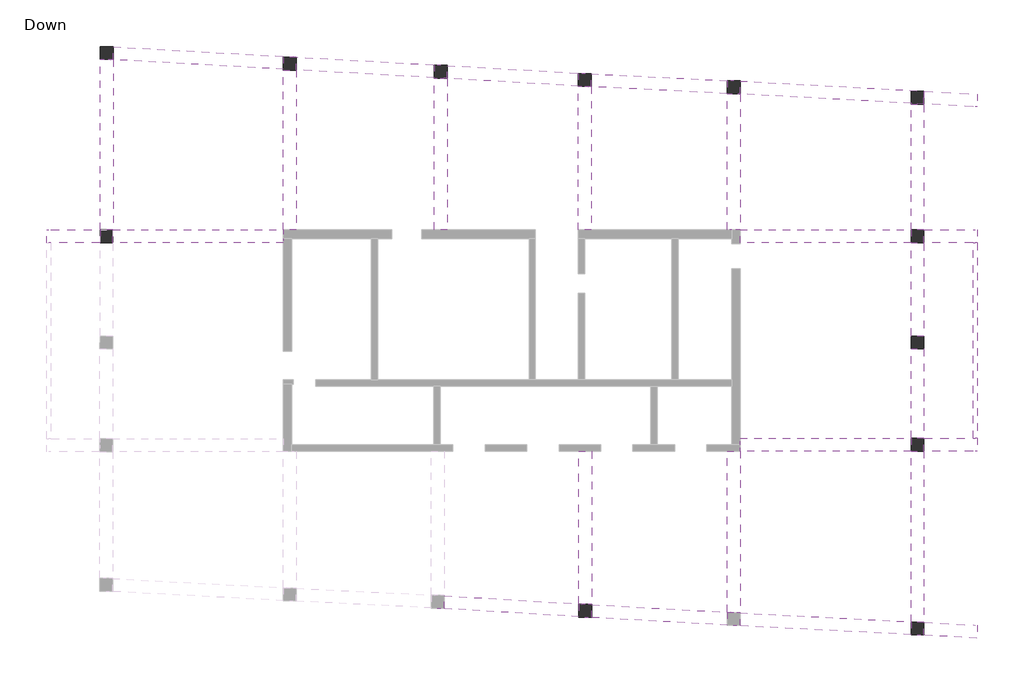
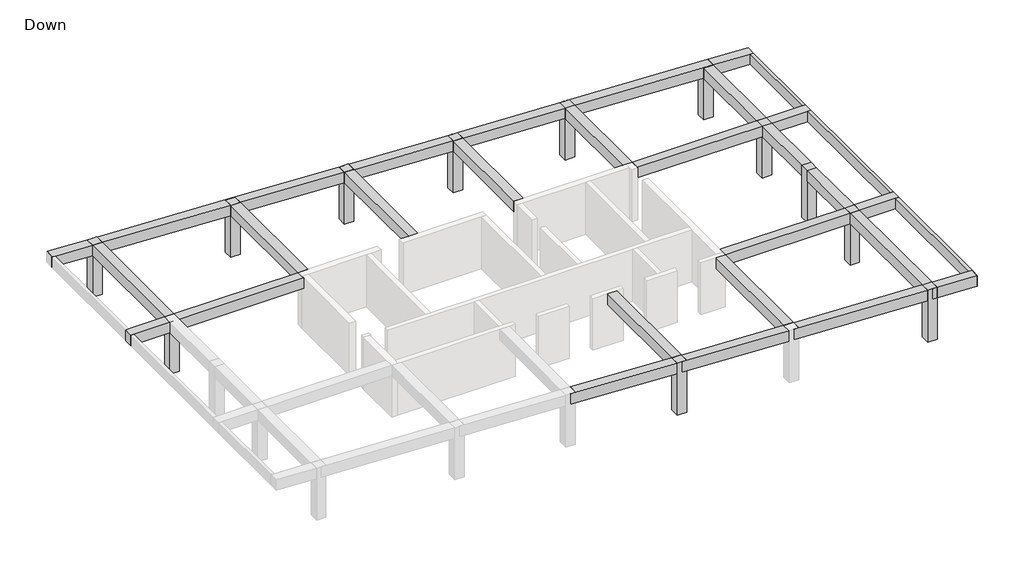
# One storey, part 2 of 2: 28 beams, 12 columns.
"""IFC4 building model written with IfcOpenShell, lengths in millimetres."""

from ifc_helpers import new_model, si_unit, origin, origin_with_axes, place, context, project, spatial, polyline, outline, extrude, faceted_brep, element, save

model = new_model("IFC4")

# Units and contexts
model_context = context("Model", 3, world=origin())
ifc_project = project(units=[si_unit("LENGTHUNIT", "METRE", prefix="MILLI")], contexts=[model_context])

# Site, building, storey
site = spatial("IfcSite", under=ifc_project)
building = spatial("IfcBuilding", under=site)
storey = spatial("IfcBuildingStorey", under=building, Name="Down", Elevation=0.0)

# Beams
placement = place(None, origin())
element("IfcBeam", 1, ObjectType="Concrete Rectengular Beam : 20/70", at=placement, inside=storey, context=model_context, shape_type="Brep", body=[
    faceted_brep([(24768.7448881, 7874.5583517, 3500.0), (24568.7448881, 7885.5038131, 3500.0), (24568.7448881, 2137.8533878, 3500.0), (24768.7448881, 2137.8533878, 3500.0), (24768.7448881, 7874.5583517, 2800.0), (24768.7448881, 2137.8533878, 2800.0), (24568.7448881, 7885.5038131, 2800.0), (24568.7448881, 2137.8533878, 2800.0), (24568.7448881, 7885.5038131, 3250.0), (24568.7448881, 2137.8533878, 3250.0)], [[[0, 1, 2, 3]], [[4, 0, 3, 5]], [[6, 4, 5, 7]], [[1, 8, 6, 7, 9, 2]], [[1, 0, 4, 6, 8]], [[3, 2, 9, 7, 5]]]),
    faceted_brep([(24768.7448881, -16893.2994445, 2800.0), (24768.7448881, -16893.2994445, 3500.0), (24737.8761026, -16891.709202, 3500.0), (24737.8761026, -16891.709202, 2800.0), (24768.7448881, -16292.5037964, 2800.0), (24768.7448881, -16292.5037964, 3500.0), (24568.7448881, -16282.2005564, 3500.0), (24568.7448881, -16282.2005564, 3250.0), (24568.7448881, -16282.2005564, 2800.0), (24568.7448881, -8172.2965545, 3500.0), (24768.7448881, -8172.2965545, 3500.0), (24768.7448881, -8172.2965545, 2800.0), (24568.7448881, -8172.2965545, 2800.0), (24568.7448881, -8172.2965545, 3250.0)], [[[0, 1, 2, 3]], [[4, 5, 6, 7, 8]], [[5, 4, 3, 2]], [[2, 1, 5]], [[0, 3, 4]], [[9, 10, 11, 12, 13]], [[6, 5, 10, 9]], [[1, 0, 4, 11, 10, 5]], [[4, 8, 12, 11]], [[8, 7, 6, 9, 13, 12]]]),
    faceted_brep([(24768.7448881, -7572.2965545, 3500.0), (24568.7448881, -7572.2965545, 3500.0), (24568.7448881, -7572.2965545, 3250.0), (24568.7448881, -7572.2965545, 2800.0), (24768.7448881, -7572.2965545, 2800.0), (24568.7448881, 1537.8533878, 3500.0), (24768.7448881, 1537.8533878, 3500.0), (24768.7448881, 1537.8533878, 2800.0), (24568.7448881, 1537.8533878, 2800.0), (24568.7448881, 1537.8533878, 3250.0)], [[[0, 1, 2, 3, 4]], [[5, 6, 7, 8, 9]], [[1, 0, 6, 5]], [[0, 4, 7, 6]], [[4, 3, 8, 7]], [[3, 2, 1, 5, 9, 8]]]),
])
element("IfcBeam", 2, ObjectType="Concrete Rectengular Beam : 60/70", at=placement, inside=storey, context=model_context, shape_type="Brep", body=[
    faceted_brep([(-15535.8201837, 10679.5964096, 3500.0), (-15536.4529131, 10091.1580694, 3500.0), (-15762.4756779, 10091.4011046, 3500.0), (-15536.4663265, 10078.6836364, 3500.0), (-7599.5626242, 9632.0768029, 3500.0), (-7599.5626242, 10196.3425232, 3500.0), (-6999.5626242, 10196.3425232, 3500.0), (-6999.5626242, 10199.2641414, 3500.0), (-7278.9210368, 10214.9835429, 3500.0), (-15762.4756779, 10091.4011046, 2800.0), (-15536.4663265, 10078.6836364, 2800.0), (-7599.5626242, 9632.0768029, 2800.0), (-7599.5626242, 9632.0768029, 3250.0), (-15536.4529131, 10091.1580694, 2800.0), (-15535.8201837, 10679.5964096, 2800.0), (-7278.9210368, 10214.9835429, 2800.0), (-6999.5626242, 10199.2641414, 2800.0), (-6999.5626242, 10196.3425232, 2800.0), (-7599.5626242, 10196.3425232, 2800.0)], [[[0, 1, 2, 3, 4, 5, 6, 7, 8]], [[2, 9, 10, 11, 12, 4, 3]], [[13, 14, 15, 16, 17, 18, 11, 10, 9]], [[14, 0, 8, 7, 16, 15]], [[1, 0, 14, 13]], [[1, 13, 9, 2]], [[5, 4, 12, 11, 18]], [[5, 18, 17, 6]], [[16, 7, 6, 17]]]),
    faceted_brep([(-16135.8074053, 10691.8028834, 2800.0), (-16135.8074053, 10691.8028834, 3500.0), (-16136.4303725, 10112.4434063, 3500.0), (-16136.4303725, 10112.4434063, 3250.0), (-16136.4303725, 10112.4434063, 2800.0), (-15745.2858019, 10691.3829677, 2800.0), (-15745.2858019, 10691.3829677, 3500.0), (-18643.7818749, 10253.5312104, 3500.0), (-18643.7818749, 10253.5312104, 2800.0), (-18443.7818749, 10242.2772794, 2800.0), (-18443.7818749, 10242.2772794, 3500.0), (-18610.0734048, 10852.5835779, 3500.0), (-18610.0734048, 10852.5835779, 2800.0)], [[[0, 1, 2, 3, 4]], [[1, 0, 5, 6]], [[7, 8, 9, 4, 3, 2, 10]], [[11, 12, 8, 7]], [[2, 1, 6, 11, 7, 10]], [[0, 4, 9, 8, 12, 5]], [[12, 11, 6, 5]]]),
])
element("IfcBeam", 3, ObjectType="Concrete Rectengular Beam : 60/70", at=placement, inside=storey, context=model_context, shape_type="Brep", body=[
    faceted_brep([(-566.8499256, 9237.1370793, 3500.0), (-566.8499256, 9820.7307485, 3500.0), (-258.416148, 9820.7307485, 3500.0), (-7278.876803, 10215.7696478, 3500.0), (-7278.9210368, 10214.9835429, 3500.0), (-6999.5626242, 10199.2641414, 3500.0), (-6999.5626242, 10196.3425232, 3500.0), (-6999.5626242, 9599.1036038, 3500.0), (-566.8499256, 9237.1370793, 2800.0), (-566.8499256, 9237.1370793, 3250.0), (-6999.5626242, 9599.1036038, 3250.0), (-6999.5626242, 9599.1036038, 2800.0), (-566.8499256, 9820.7307485, 2800.0), (-6999.5626242, 10196.3425232, 2800.0), (-6999.5626242, 10199.2641414, 2800.0), (-7278.9210368, 10214.9835429, 2800.0), (-7278.876803, 10215.7696478, 2800.0), (-258.416148, 9820.7307485, 2800.0)], [[[0, 1, 2, 3, 4, 5, 6, 7]], [[8, 9, 0, 7, 10, 11]], [[12, 8, 11, 13, 14, 15, 16, 17]], [[2, 17, 16, 3]], [[12, 1, 0, 9, 8]], [[1, 12, 17, 2]], [[3, 16, 15, 4]], [[5, 14, 13, 11, 10, 7, 6]], [[14, 5, 4, 15]]]),
])
element("IfcBeam", 4, ObjectType="Concrete Rectengular Beam : 60/70", at=placement, inside=storey, context=model_context, shape_type="Brep", body=[
    faceted_brep([(33.1500744, 9803.9611146, 3500.0), (33.1500744, 9220.7307485, 3500.0), (-275.4758313, 9220.7307485, 3500.0), (33.1500744, 9202.9682104, 3500.0), (6156.4488056, 8850.5502029, 3500.0), (6156.4488056, 9432.8840986, 3500.0), (6480.6509764, 9432.8840986, 3500.0), (-275.4758313, 9220.7307485, 2800.0), (33.1500744, 9202.9682104, 2800.0), (6156.4488056, 8850.5502029, 2800.0), (6156.4488056, 8850.5502029, 3300.0), (33.1500744, 9220.7307485, 2800.0), (33.1500744, 9803.9611146, 2800.0), (6480.6509764, 9432.8840986, 2800.0), (6156.4488056, 9432.8840986, 2800.0)], [[[0, 1, 2, 3, 4, 5, 6]], [[2, 7, 8, 9, 10, 4, 3]], [[11, 12, 13, 14, 9, 8, 7]], [[12, 0, 6, 13]], [[11, 1, 0, 12]], [[1, 11, 7, 2]], [[14, 5, 4, 10, 9]], [[5, 14, 13, 6]]]),
])
element("IfcBeam", 5, ObjectType="Concrete Rectengular Beam : 60/70", at=placement, inside=storey, context=model_context, shape_type="Brep", body=[
    faceted_brep([(6756.4488056, 9419.0415842, 3500.0), (6756.4488056, 8832.8840986, 3500.0), (6464.5319229, 8832.8840986, 3500.0), (6756.4488056, 8818.2924867, 3500.0), (13105.5837537, 8500.9277886, 3500.0), (13105.5837537, 9086.6836559, 3500.0), (13405.5353315, 9086.6836559, 3500.0), (6464.5319229, 8832.8840986, 2800.0), (6756.4488056, 8818.2924867, 2800.0), (13105.5837537, 8500.9277886, 2800.0), (13105.5837537, 8500.9277886, 3300.0), (6756.4488056, 8832.8840986, 2800.0), (6756.4488056, 9419.0415842, 2800.0), (13405.5353315, 9086.6836559, 2800.0), (13105.5837537, 9086.6836559, 2800.0)], [[[0, 1, 2, 3, 4, 5, 6]], [[2, 7, 8, 9, 10, 4, 3]], [[11, 12, 13, 14, 9, 8, 7]], [[12, 0, 6, 13]], [[11, 1, 0, 12]], [[1, 11, 7, 2]], [[14, 5, 4, 10, 9]], [[5, 14, 13, 6]]]),
])
element("IfcBeam", 6, ObjectType="Concrete Rectengular Beam : 60/70", at=placement, inside=storey, context=model_context, shape_type="Brep", body=[
    faceted_brep([(13705.5837537, 9080.9132195, 3500.0), (13705.5837537, 8486.6836559, 3500.0), (13583.7380368, 8486.6836559, 3500.0), (13705.5837537, 8480.0153679, 3500.0), (21672.320563, 8044.0173164, 3500.0), (21672.6744767, 8043.9979477, 3500.0), (22272.320563, 8011.1809322, 3500.0), (22272.320563, 8612.0787839, 3500.0), (13583.7380368, 8486.6836559, 2800.0), (13705.5837537, 8480.0153679, 2800.0), (21672.320563, 8044.0173164, 2800.0), (21672.6744767, 8043.9979477, 2800.0), (22272.320563, 8011.1809322, 2800.0), (13705.5837537, 8486.6836559, 2800.0), (13705.5837537, 9080.9132195, 2800.0), (22272.320563, 8612.0787839, 2800.0)], [[[0, 1, 2, 3, 4, 5, 6, 7]], [[2, 8, 9, 10, 11, 12, 6, 5, 4, 3]], [[13, 14, 15, 12, 11, 10, 9, 8]], [[14, 0, 7, 15]], [[13, 1, 0, 14]], [[1, 13, 8, 2]], [[7, 6, 12, 15]]]),
    faceted_brep([(13415.7050313, 9096.7775014, 3500.0), (13415.7050313, 9096.7775014, 2800.0), (13415.1526223, 9086.6836559, 2800.0), (13415.1526223, 9086.6836559, 3500.0), (13600.1439538, 9086.6836559, 3500.0), (13600.1439538, 9086.6836559, 2800.0)], [[[0, 1, 2, 3]], [[4, 3, 2, 5]], [[0, 3, 4]], [[2, 1, 5]], [[1, 0, 4, 5]]]),
])
element("IfcBeam", 7, ObjectType="Concrete Rectengular Beam : 60/70", at=placement, inside=storey, context=model_context, shape_type="Brep", body=[
    faceted_brep([(24768.7448881, 7874.5583517, 3500.0), (24768.7448881, 8475.4562033, 3500.0), (22272.320563, 8612.0787839, 3500.0), (22272.320563, 8011.1809322, 3500.0), (22272.7208607, 8011.159025, 3500.0), (24568.7448881, 7885.5038131, 3500.0), (24768.7448881, 7874.5583517, 2800.0), (22272.320563, 8011.1809322, 2800.0), (24568.7448881, 7885.5038131, 2800.0), (24768.7448881, 8475.4562033, 2800.0), (22272.320563, 8612.0787839, 2800.0)], [[[0, 1, 2, 3, 4, 5]], [[6, 0, 5, 4, 3, 7, 8]], [[9, 6, 8, 7, 10]], [[1, 9, 10, 2]], [[1, 0, 6, 9]], [[3, 2, 10, 7]]]),
])
element("IfcBeam", 8, ObjectType="Concrete Rectengular Beam : 60/70", at=placement, inside=storey, context=model_context, shape_type="Brep", body=[
    faceted_brep([(21672.320563, 2137.8533878, 3500.0), (22272.320563, 2137.8533878, 3500.0), (22272.320563, 7998.3813629, 3500.0), (21672.7392644, 7997.5451268, 3500.0), (21672.6744767, 8043.9979477, 3500.0), (21672.320563, 8044.0173164, 3500.0), (21672.320563, 2137.8533878, 2800.0), (21672.320563, 2137.8533878, 3250.0), (21672.320563, 8044.0173164, 3250.0), (21672.320563, 8044.0173164, 2800.0), (22272.320563, 2137.8533878, 2800.0), (21672.6744767, 8043.9979477, 2800.0), (21672.7392644, 7997.5451268, 2800.0), (22272.320563, 7998.3813629, 2800.0), (22272.320563, 2137.8533878, 3250.0), (22272.320563, 7998.3813629, 3250.0)], [[[0, 1, 2, 3, 4, 5]], [[6, 7, 0, 5, 8, 9]], [[10, 6, 9, 11, 12, 13]], [[1, 14, 10, 13, 15, 2]], [[1, 0, 7, 6, 10, 14]], [[9, 8, 5, 4, 11]], [[12, 3, 2, 15, 13]], [[3, 12, 11, 4]]]),
])
element("IfcBeam", 9, ObjectType="Concrete Rectengular Beam : 60/70", at=placement, inside=storey, context=model_context, shape_type="Brep", body=[
    faceted_brep([(21672.320563, -2812.4954615, 3500.0), (22272.320563, -2812.4954615, 3500.0), (22272.320563, 1537.8533878, 3500.0), (21672.320563, 1537.8533878, 3500.0), (21672.320563, -2812.4954615, 2800.0), (21672.320563, 1537.8533878, 3250.0), (21672.320563, 1537.8533878, 2800.0), (22272.320563, -2812.4954615, 2800.0), (22272.320563, 1537.8533878, 2800.0), (22272.320563, 1537.8533878, 3250.0)], [[[0, 1, 2, 3]], [[4, 0, 3, 5, 6]], [[7, 4, 6, 8]], [[1, 7, 8, 9, 2]], [[1, 0, 4, 7]], [[3, 2, 9, 8, 6, 5]]]),
])
element("IfcBeam", 10, ObjectType="Concrete Rectengular Beam : 60/70", at=placement, inside=storey, context=model_context, shape_type="Brep", body=[
    faceted_brep([(22272.320563, -3412.4954615, 3500.0), (21672.320563, -3412.4954615, 3500.0), (21672.320563, -7572.2965545, 3500.0), (22272.320563, -7572.2965545, 3500.0), (21672.320563, -3412.4954615, 2800.0), (21672.320563, -7572.2965545, 2800.0), (21672.320563, -7572.2965545, 3250.0), (22272.320563, -3412.4954615, 2800.0), (22272.320563, -7572.2965545, 2800.0), (22272.320563, -7572.2965545, 3250.0)], [[[0, 1, 2, 3]], [[1, 4, 5, 6, 2]], [[4, 7, 8, 5]], [[7, 0, 3, 9, 8]], [[1, 0, 7, 4]], [[3, 2, 6, 5, 8, 9]]]),
])
element("IfcBeam", 11, ObjectType="Concrete Rectengular Beam : 60/70", at=placement, inside=storey, context=model_context, shape_type="Brep", body=[
    faceted_brep([(21672.320563, -16148.8404655, 3500.0), (22272.320563, -16148.8404655, 3500.0), (22272.320563, -8172.2965545, 3500.0), (21672.320563, -8172.2965545, 3500.0), (21672.320563, -16132.9877815, 3500.0), (21672.320563, -16148.8404655, 2800.0), (21672.320563, -8172.2965545, 3250.0), (21672.320563, -8172.2965545, 2800.0), (21672.320563, -16132.9877815, 2800.0), (22272.320563, -16148.8404655, 2800.0), (22272.320563, -8172.2965545, 2800.0), (22272.320563, -8172.2965545, 3250.0)], [[[0, 1, 2, 3, 4]], [[5, 0, 4, 3, 6, 7, 8]], [[9, 5, 8, 7, 10]], [[1, 9, 10, 11, 2]], [[1, 0, 5, 9]], [[3, 2, 11, 10, 7, 6]]]),
])
element("IfcBeam", 12, ObjectType="Concrete Rectengular Beam : 60/70", at=placement, inside=storey, context=model_context, shape_type="Brep", body=[
    faceted_brep([(21672.320563, -16733.7834296, 3500.0), (21672.320563, -16148.8404655, 3500.0), (21672.320563, -16132.9877815, 3500.0), (13705.5837537, -15722.5717744, 3500.0), (13698.0421838, -15722.1832613, 3500.0), (13698.0421838, -16307.1262254, 3500.0), (13390.319874, -16307.1262254, 3500.0), (21672.320563, -16132.9877815, 2800.0), (13705.5837537, -15722.5717744, 2800.0), (13698.0421838, -15722.1832613, 2800.0), (21672.320563, -16132.9877815, 3250.0), (21672.320563, -16148.8404655, 2800.0), (21672.320563, -16733.7834296, 2800.0), (13390.319874, -16307.1262254, 2800.0), (13698.0421838, -16307.1262254, 2800.0)], [[[0, 1, 2, 3, 4, 5, 6]], [[7, 8, 9, 4, 3, 2, 10]], [[7, 11, 12, 13, 14, 9, 8]], [[12, 0, 6, 13]], [[0, 12, 11, 7, 10, 2, 1]], [[14, 5, 4, 9]], [[5, 14, 13, 6]]]),
])
element("IfcBeam", 13, ObjectType="Concrete Rectengular Beam : 60/70", at=placement, inside=storey, context=model_context, shape_type="Brep", body=[
    faceted_brep([(13098.0421838, -16290.7966787, 3500.0), (13098.0421838, -15707.1262254, 3500.0), (13406.4353858, -15707.1262254, 3500.0), (13105.5837537, -15690.2789818, 3500.0), (6772.0250706, -15335.6091222, 3500.0), (6772.0250706, -15919.2795755, 3500.0), (6463.6318687, -15919.2795755, 3500.0), (13406.4353858, -15707.1262254, 2800.0), (13105.5837537, -15690.2789818, 2800.0), (6772.0250706, -15335.6091222, 2800.0), (6772.0250706, -15335.6091222, 3250.0), (13098.0421838, -15707.1262254, 2800.0), (13098.0421838, -16290.7966787, 2800.0), (6463.6318687, -15919.2795755, 2800.0), (6772.0250706, -15919.2795755, 2800.0)], [[[0, 1, 2, 3, 4, 5, 6]], [[2, 7, 8, 9, 10, 4, 3]], [[11, 12, 13, 14, 9, 8, 7]], [[12, 0, 6, 13]], [[11, 1, 0, 12]], [[1, 11, 7, 2]], [[14, 5, 4, 10, 9]], [[5, 14, 13, 6]]]),
])
element("IfcBeam", 14, ObjectType="Concrete Rectengular Beam : 60/70", at=placement, inside=storey, context=model_context, shape_type="Brep", body=[
    faceted_brep([(6172.0250706, -15901.5041134, 3500.0), (6172.0250706, -15319.2795755, 3500.0), (6481.1841464, -15319.2795755, 3500.0), (6172.0250706, -15300.3845543, 3500.0), (-102.7226745, -14916.8878336, 3500.0), (-102.7226745, -15499.1123715, 3500.0), (-411.8817502, -15499.1123715, 3500.0), (6481.1841464, -15319.2795755, 2800.0), (6172.0250706, -15300.3845543, 2800.0), (-102.7226745, -14916.8878336, 2800.0), (-102.7226745, -14916.8878336, 3300.0), (6172.0250706, -15319.2795755, 2800.0), (6172.0250706, -15901.5041134, 2800.0), (-411.8817502, -15499.1123715, 2800.0), (-102.7226745, -15499.1123715, 2800.0)], [[[0, 1, 2, 3, 4, 5, 6]], [[2, 7, 8, 9, 10, 4, 3]], [[11, 12, 13, 14, 9, 8, 7]], [[12, 0, 6, 13]], [[11, 1, 0, 12]], [[1, 11, 7, 2]], [[14, 5, 4, 10, 9]], [[5, 14, 13, 6]]]),
])
element("IfcBeam", 15, ObjectType="Concrete Rectengular Beam : 60/70", at=placement, inside=storey, context=model_context, shape_type="Brep", body=[
    faceted_brep([(-16145.0052005, 2137.8533878, 3500.0), (-15545.0048536, 2137.8533878, 3500.0), (-15536.4663265, 10078.6836364, 3500.0), (-15762.4756779, 10091.4011046, 3500.0), (-16136.4525662, 10091.8032303, 3500.0), (-15545.0048536, 2137.8533878, 3250.0), (-15545.0048536, 2137.8533878, 2800.0), (-15536.4663265, 10078.6836364, 2800.0), (-15536.4663265, 10078.6836364, 3250.0), (-16145.0052005, 2137.8533878, 2800.0), (-16136.4525662, 10091.8032303, 2800.0), (-15762.4756779, 10091.4011046, 2800.0), (-16136.4525662, 10091.8032303, 3250.0), (-16145.0052005, 2137.8533878, 3250.0)], [[[0, 1, 2, 3, 4]], [[2, 1, 5, 6, 7, 8]], [[6, 9, 10, 11, 7]], [[0, 4, 12, 10, 9, 13]], [[4, 3, 11, 10, 12]], [[3, 2, 8, 7, 11]], [[1, 0, 13, 9, 6, 5]]]),
])
element("IfcBeam", 16, ObjectType="Concrete Rectengular Beam : 60/70", at=placement, inside=storey, context=model_context, shape_type="Brep", body=[
    faceted_brep([(22272.320563, -7572.2965545, 3500.0), (22272.320563, -8172.2965545, 3500.0), (24568.7448881, -8172.2965545, 3500.0), (24768.7448881, -8172.2965545, 3500.0), (24768.7448881, -7572.2965545, 3500.0), (24568.7448881, -7572.2965545, 3500.0), (24768.7448881, -8172.2965545, 2800.0), (22272.320563, -8172.2965545, 3250.0), (22272.320563, -8172.2965545, 2800.0), (24568.7448881, -8172.2965545, 2800.0), (22272.320563, -7572.2965545, 2800.0), (24568.7448881, -7572.2965545, 2800.0), (24768.7448881, -7572.2965545, 2800.0), (22272.320563, -7572.2965545, 3250.0)], [[[0, 1, 2, 3, 4, 5]], [[6, 3, 2, 1, 7, 8, 9]], [[8, 10, 11, 12, 6, 9]], [[10, 13, 0, 5, 4, 12, 11]], [[0, 13, 10, 8, 7, 1]], [[4, 3, 6, 12]]]),
])
element("IfcBeam", 17, ObjectType="Concrete Rectengular Beam : 60/70", at=placement, inside=storey, context=model_context, shape_type="Brep", body=[
    faceted_brep([(21964.5982532, -16748.8404655, 3500.0), (24737.8761026, -16891.709202, 3500.0), (24768.7448881, -16292.5037964, 3500.0), (24568.7448881, -16282.2005564, 3500.0), (22272.320563, -16163.8975015, 3500.0), (22272.320563, -16748.8404655, 3500.0), (21964.5982532, -16748.8404655, 2800.0), (24737.8761026, -16891.709202, 2800.0), (22272.320563, -16163.8975015, 2800.0), (24568.7448881, -16282.2005564, 2800.0), (24768.7448881, -16292.5037964, 2800.0), (22272.320563, -16748.8404655, 2800.0), (22272.320563, -16163.8975015, 3250.0)], [[[0, 1, 2, 3, 4, 5]], [[1, 0, 6, 7]], [[8, 9, 10, 7, 6, 11]], [[10, 9, 8, 12, 4, 3, 2]], [[11, 5, 4, 12, 8]], [[5, 11, 6, 0]], [[2, 1, 7, 10]]]),
])
element("IfcBeam", 18, ObjectType="Concrete Rectengular Beam : 60/70", at=placement, inside=storey, context=model_context, shape_type="Brep", body=[
    faceted_brep([(22272.320563, 2137.8533878, 3500.0), (22272.320563, 1537.8533878, 3500.0), (24568.7448881, 1537.8533878, 3500.0), (24768.7448881, 1537.8533878, 3500.0), (24768.7448881, 2137.8533878, 3500.0), (24568.7448881, 2137.8533878, 3500.0), (24768.7448881, 1537.8533878, 2800.0), (22272.320563, 1537.8533878, 3250.0), (22272.320563, 1537.8533878, 2800.0), (24568.7448881, 1537.8533878, 2800.0), (22272.320563, 2137.8533878, 2800.0), (24568.7448881, 2137.8533878, 2800.0), (24768.7448881, 2137.8533878, 2800.0), (22272.320563, 2137.8533878, 3250.0)], [[[0, 1, 2, 3, 4, 5]], [[6, 3, 2, 1, 7, 8, 9]], [[8, 10, 11, 12, 6, 9]], [[10, 13, 0, 5, 4, 12, 11]], [[0, 13, 10, 8, 7, 1]], [[4, 3, 6, 12]]]),
])
element("IfcBeam", 19, ObjectType="Concrete Rectengular Beam : 60/70", at=placement, inside=storey, context=model_context, shape_type="Brep", body=[
    faceted_brep([(-16145.6503618, 1537.8533878, 3500.0), (-16145.0052005, 2137.8533878, 3500.0), (-18443.7818749, 2137.8533878, 3500.0), (-18643.7818749, 2137.8533878, 3500.0), (-18643.7818749, 1537.8533878, 3500.0), (-18443.7818749, 1537.8533878, 3500.0), (-18643.7818749, 2137.8533878, 2800.0), (-16145.0052005, 2137.8533878, 3250.0), (-16145.0052005, 2137.8533878, 2800.0), (-18443.7818749, 2137.8533878, 2800.0), (-16145.6503618, 1537.8533878, 2800.0), (-18443.7818749, 1537.8533878, 2800.0), (-18643.7818749, 1537.8533878, 2800.0), (-16145.6503618, 1537.8533878, 3250.0)], [[[0, 1, 2, 3, 4, 5]], [[6, 3, 2, 1, 7, 8, 9]], [[8, 10, 11, 12, 6, 9]], [[10, 13, 0, 5, 4, 12, 11]], [[1, 0, 13, 10, 8, 7]], [[4, 3, 6, 12]]]),
])
element("IfcBeam", 20, ObjectType="Concrete Rectengular Beam : 60/70", at=placement, inside=storey, context=model_context, shape_type="Brep", body=[
    faceted_brep([(-15545.0048536, 2137.8533878, 3500.0), (-15545.6500149, 1537.8533878, 3500.0), (-7599.5626242, 1537.8533878, 3500.0), (-7599.5626242, 1737.8533878, 3500.0), (-7599.5626242, 2137.8533878, 3500.0), (-15545.6500149, 1537.8533878, 3250.0), (-15545.6500149, 1537.8533878, 2800.0), (-7599.5626242, 1537.8533878, 2800.0), (-7599.5626242, 1537.8533878, 3250.0), (-15545.0048536, 2137.8533878, 2800.0), (-7599.5626242, 2137.8533878, 2800.0), (-15545.0048536, 2137.8533878, 3250.0), (-7599.5626242, 2137.8533878, 3250.0)], [[[0, 1, 2, 3, 4]], [[1, 5, 6, 7, 8, 2]], [[6, 9, 10, 7]], [[9, 11, 0, 4, 12, 10]], [[1, 0, 11, 9, 6, 5]], [[2, 8, 7, 10, 12, 4, 3]]]),
])
element("IfcBeam", 21, ObjectType="Concrete Rectengular Beam : 60/70", at=placement, inside=storey, context=model_context, shape_type="Brep", body=[
    faceted_brep([(-6999.5626242, 9596.3425232, 3500.0), (-7599.5626242, 9596.3425232, 3500.0), (-7599.5626242, 2137.8533878, 3500.0), (-6999.5626242, 2137.8533878, 3500.0), (-7599.5626242, 2137.8533878, 2800.0), (-7599.5626242, 2137.8533878, 3250.0), (-7599.5626242, 9596.3425232, 2800.0), (-6999.5626242, 9596.3425232, 2800.0), (-6999.5626242, 2137.8533878, 2800.0), (-6999.5626242, 2137.8533878, 3250.0)], [[[0, 1, 2, 3]], [[4, 5, 2, 1, 6]], [[6, 7, 8, 4]], [[3, 9, 8, 7, 0]], [[1, 0, 7, 6]], [[3, 2, 5, 4, 8, 9]]]),
])
element("IfcBeam", 22, ObjectType="Concrete Rectengular Beam : 60/70", at=placement, inside=storey, context=model_context, shape_type="Brep", body=[
    faceted_brep([(-566.8499256, 9220.7307485, 3500.0), (-566.8499256, 2137.8533878, 3500.0), (33.1500744, 2137.8533878, 3500.0), (33.1500744, 9202.9682104, 3500.0), (-275.4758313, 9220.7307485, 3500.0), (-566.8499256, 9220.7307485, 2800.0), (-566.8499256, 2137.8533878, 2800.0), (-566.8499256, 2137.8533878, 3250.0), (-275.4758313, 9220.7307485, 2800.0), (33.1500744, 9202.9682104, 2800.0), (33.1500744, 2137.8533878, 2800.0), (33.1500744, 2137.8533878, 3300.0), (33.1500744, 9202.9682104, 3300.0)], [[[0, 1, 2, 3, 4]], [[0, 5, 6, 7, 1]], [[6, 5, 8, 9, 10]], [[2, 11, 10, 9, 12, 3]], [[5, 0, 4, 8]], [[2, 1, 7, 6, 10, 11]], [[4, 3, 12, 9, 8]]]),
])
element("IfcBeam", 23, ObjectType="Concrete Rectengular Beam : 60/70", at=placement, inside=storey, context=model_context, shape_type="Brep", body=[
    faceted_brep([(6756.4488056, 8818.2924867, 3500.0), (6464.5319229, 8832.8840986, 3500.0), (6156.4488056, 8832.8840986, 3500.0), (6156.4488056, 2137.8533878, 3500.0), (6756.4488056, 2137.8533878, 3500.0), (6156.4488056, 8832.8840986, 2800.0), (6156.4488056, 2137.8533878, 2800.0), (6156.4488056, 2137.8533878, 3300.0), (6464.5319229, 8832.8840986, 2800.0), (6756.4488056, 8818.2924867, 2800.0), (6756.4488056, 2137.8533878, 2800.0), (6756.4488056, 8818.2924867, 3300.0), (6756.4488056, 2137.8533878, 3300.0)], [[[0, 1, 2, 3, 4]], [[2, 5, 6, 7, 3]], [[8, 9, 10, 6, 5]], [[9, 11, 0, 4, 12, 10]], [[0, 11, 9, 8, 1]], [[2, 1, 8, 5]], [[4, 3, 7, 6, 10, 12]]]),
])
element("IfcBeam", 24, ObjectType="Concrete Rectengular Beam : 60/70", at=placement, inside=storey, context=model_context, shape_type="Brep", body=[
    faceted_brep([(13105.5837537, 8486.6836559, 3500.0), (13105.5837537, 8486.6836559, 2800.0), (13105.5837537, 2137.8533878, 2800.0), (13105.5837537, 2137.8533878, 3300.0), (13105.5837537, 2137.8533878, 3500.0), (13705.5837537, 8480.0153679, 2800.0), (13705.5837537, 8480.0153679, 3250.0), (13705.5837537, 8480.0153679, 3500.0), (13705.5837537, 2137.8533878, 3500.0), (13705.5837537, 2137.8533878, 3250.0), (13705.5837537, 2137.8533878, 2800.0), (13583.7380368, 8486.6836559, 2800.0), (13583.7380368, 8486.6836559, 3500.0), (13305.5837537, 2137.8533878, 3500.0)], [[[0, 1, 2, 3, 4]], [[5, 6, 7, 8, 9, 10]], [[7, 6, 5, 11, 12]], [[7, 12, 0, 4, 13, 8]], [[11, 5, 10, 2, 1]], [[1, 0, 12, 11]], [[4, 3, 2, 10, 9, 8, 13]]]),
])
element("IfcBeam", 25, ObjectType="Concrete Rectengular Beam : 60/70", at=placement, inside=storey, context=model_context, shape_type="Brep", body=[
    faceted_brep([(21672.320563, 1537.8533878, 3500.0), (21672.320563, 2137.8533878, 3500.0), (13705.5837537, 2137.8533878, 3500.0), (13705.5837537, 1537.8533878, 3500.0), (21672.320563, 2137.8533878, 3250.0), (21672.320563, 2137.8533878, 2800.0), (13705.5837537, 2137.8533878, 2800.0), (13705.5837537, 2137.8533878, 3250.0), (21672.320563, 1537.8533878, 2800.0), (13705.5837537, 1537.8533878, 2800.0), (21672.320563, 1537.8533878, 3250.0), (13705.5837537, 1537.8533878, 3250.0)], [[[0, 1, 2, 3]], [[1, 4, 5, 6, 7, 2]], [[5, 8, 9, 6]], [[8, 10, 0, 3, 11, 9]], [[5, 4, 1, 0, 10, 8]], [[3, 2, 7, 6, 9, 11]]]),
])
element("IfcBeam", 26, ObjectType="Concrete Rectengular Beam : 60/70", at=placement, inside=storey, context=model_context, shape_type="Brep", body=[
    faceted_brep([(13705.5837537, -7572.2965545, 3500.0), (13705.5837537, -7872.2965545, 3500.0), (13705.5837537, -8172.2965545, 3500.0), (21672.320563, -8172.2965545, 3500.0), (21672.320563, -7572.2965545, 3500.0), (21672.320563, -7572.2965545, 3250.0), (21672.320563, -7572.2965545, 2800.0), (13705.5837537, -7572.2965545, 2800.0), (13705.5837537, -7572.2965545, 3250.0), (13705.5837537, -8172.2965545, 2800.0), (21672.320563, -8172.2965545, 2800.0), (21672.320563, -8172.2965545, 3250.0), (13705.5837537, -8172.2965545, 3250.0)], [[[0, 1, 2, 3, 4]], [[4, 5, 6, 7, 8, 0]], [[9, 7, 6, 10]], [[10, 11, 3, 2, 12, 9]], [[6, 5, 4, 3, 11, 10]], [[0, 8, 7, 9, 12, 2, 1]]]),
])
element("IfcBeam", 27, ObjectType="Concrete Rectengular Beam : 60/70", at=placement, inside=storey, context=model_context, shape_type="Brep", body=[
    faceted_brep([(13698.0421838, -15707.1262254, 3500.0), (13698.0421838, -15722.1832613, 3500.0), (13705.5837537, -15722.5717744, 3500.0), (13705.5837537, -8172.2965545, 3500.0), (13105.5837537, -8172.2965545, 3500.0), (13105.5837537, -15690.2789818, 3500.0), (13406.4353858, -15707.1262254, 3500.0), (13705.5837537, -15722.5717744, 3250.0), (13705.5837537, -15722.5717744, 2800.0), (13705.5837537, -8172.2965545, 2800.0), (13705.5837537, -8172.2965545, 3250.0), (13698.0421838, -15722.1832613, 2800.0), (13698.0421838, -15707.1262254, 2800.0), (13406.4353858, -15707.1262254, 2800.0), (13105.5837537, -15690.2789818, 2800.0), (13105.5837537, -8172.2965545, 2800.0), (13105.5837537, -8172.2965545, 3250.0), (13105.5837537, -15690.2789818, 3250.0)], [[[0, 1, 2, 3, 4, 5, 6]], [[2, 7, 8, 9, 10, 3]], [[11, 12, 13, 14, 15, 9, 8]], [[4, 16, 15, 14, 17, 5]], [[8, 7, 2, 1, 11]], [[0, 12, 11, 1]], [[12, 0, 6, 13]], [[4, 3, 10, 9, 15, 16]], [[6, 5, 17, 14, 13]]]),
])
element("IfcBeam", 28, ObjectType="Concrete Rectengular Beam : 60/70", at=placement, inside=storey, context=model_context, shape_type="Brep", body=[
    faceted_brep([(6772.0250706, -15319.2795755, 3500.0), (6772.0250706, -8172.2965545, 3500.0), (6172.0250706, -8172.2965545, 3500.0), (6172.0250706, -15300.3845543, 3500.0), (6481.1841464, -15319.2795755, 3500.0), (6772.0250706, -15319.2795755, 2800.0), (6772.0250706, -8172.2965545, 2800.0), (6772.0250706, -8172.2965545, 3250.0), (6481.1841464, -15319.2795755, 2800.0), (6172.0250706, -15300.3845543, 2800.0), (6172.0250706, -8172.2965545, 2800.0), (6172.0250706, -8172.2965545, 3300.0), (6172.0250706, -15300.3845543, 3300.0)], [[[0, 1, 2, 3, 4]], [[0, 5, 6, 7, 1]], [[6, 5, 8, 9, 10]], [[2, 11, 10, 9, 12, 3]], [[5, 0, 4, 8]], [[2, 1, 7, 6, 10, 11]], [[4, 3, 12, 9, 8]]]),
])

# Columns
element("IfcColumn", 29, ObjectType="Concrete Rectengular Column : 60/60", at=placement, inside=storey, context=model_context, shape_type="Brep", body=[
    faceted_brep([(33.1500744, 9820.7307485, 0.0), (33.1500744, 9220.7307485, 0.0), (-566.8499256, 9220.7307485, 0.0), (-566.8499256, 9820.7307485, 0.0), (33.1500744, 9820.7307485, 3500.0), (33.1500744, 9220.7307485, 3500.0), (-566.8499256, 9220.7307485, 3500.0), (-566.8499256, 9237.1370793, 3500.0), (-566.8499256, 9820.7307485, 3500.0)], [[[0, 1, 2, 3]], [[4, 5, 1, 0]], [[5, 6, 2, 1]], [[6, 7, 8, 3, 2]], [[8, 4, 0, 3]], [[4, 8, 7, 6, 5]]]),
])
element("IfcColumn", 30, ObjectType="Concrete Rectengular Column : 60/60", at=placement, inside=storey, context=model_context, shape_type="Brep", body=[
    faceted_brep([(6756.4488056, 9432.8840986, 0.0), (6756.4488056, 8832.8840986, 0.0), (6156.4488056, 8832.8840986, 0.0), (6156.4488056, 9432.8840986, 0.0), (6756.4488056, 9432.8840986, 3500.0), (6756.4488056, 8832.8840986, 3500.0), (6156.4488056, 8832.8840986, 3500.0), (6156.4488056, 8850.5502029, 3500.0), (6156.4488056, 9432.8840986, 3500.0)], [[[0, 1, 2, 3]], [[4, 5, 1, 0]], [[5, 6, 2, 1]], [[6, 7, 8, 3, 2]], [[8, 4, 0, 3]], [[4, 8, 7, 6, 5]]]),
])
element("IfcColumn", 31, ObjectType="Concrete Rectengular Column : 60/60", at=placement, inside=storey, context=model_context, shape_type="Brep", body=[
    faceted_brep([(-6999.5626242, 9596.3425232, 0.0), (-7599.5626242, 9596.3425232, 0.0), (-7599.5626242, 10196.3425232, 0.0), (-6999.5626242, 10196.3425232, 0.0), (-6999.5626242, 9596.3425232, 3500.0), (-7599.5626242, 9596.3425232, 3500.0), (-7599.5626242, 9632.0768029, 3500.0), (-7599.5626242, 10196.3425232, 3500.0), (-6999.5626242, 10196.3425232, 3500.0), (-6999.5626242, 9599.1036038, 3500.0)], [[[0, 1, 2, 3]], [[4, 5, 1, 0]], [[5, 6, 7, 2, 1]], [[7, 8, 3, 2]], [[8, 9, 4, 0, 3]], [[4, 9, 8, 7, 6, 5]]]),
])
element("IfcColumn", 32, ObjectType="Concrete Rectengular Column : 60/60", at=placement, inside=storey, context=model_context, shape_type="Brep", body=[
    faceted_brep([(-15535.8077522, 10691.1577225, 0.0), (-15536.4529131, 10091.1580694, 0.0), (-16136.4525662, 10091.8032303, 0.0), (-16135.8074053, 10691.8028834, 0.0), (-15535.8077522, 10691.1577225, 3500.0), (-15536.4529131, 10091.1580694, 3500.0), (-16136.4525662, 10091.8032303, 3500.0), (-16136.4303725, 10112.4434063, 3500.0), (-16135.8074053, 10691.8028834, 3500.0)], [[[0, 1, 2, 3]], [[4, 5, 1, 0]], [[5, 6, 2, 1]], [[6, 7, 8, 3, 2]], [[8, 4, 0, 3]], [[4, 8, 7, 6, 5]]]),
])
element("IfcColumn", 33, ObjectType="Concrete Rectengular Column : 60/60", at=placement, inside=storey, context=model_context, shape_type="Brep", body=[
    faceted_brep([(-15545.0119134, 2137.8533878, 0.0), (-15545.0119134, 1537.8533878, 0.0), (-16145.0119134, 1537.8533878, 0.0), (-16145.0119134, 2137.8533878, 0.0), (-15545.0119134, 2137.8533878, 3500.0), (-15545.0119134, 1537.8533878, 3500.0), (-15545.6500149, 1537.8533878, 3500.0), (-16145.0119134, 1537.8533878, 3500.0), (-16145.0119134, 2137.8533878, 3500.0)], [[[0, 1, 2, 3]], [[4, 5, 1, 0]], [[5, 6, 7, 2, 1]], [[7, 8, 3, 2]], [[8, 4, 0, 3]], [[4, 8, 7, 6, 5]]]),
])
element("IfcColumn", 34, ObjectType="Concrete Rectengular Column : 60/60", at=placement, inside=storey, context=model_context, shape_type="Brep", body=[
    faceted_brep([(13705.5837537, 9086.6836559, 0.0), (13705.5837537, 8486.6836559, 0.0), (13105.5837537, 8486.6836559, 0.0), (13105.5837537, 9086.6836559, 0.0), (13705.5837537, 9086.6836559, 3500.0), (13705.5837537, 8486.6836559, 3500.0), (13105.5837537, 8486.6836559, 3500.0), (13105.5837537, 8500.9277886, 3500.0), (13105.5837537, 9086.6836559, 3500.0)], [[[0, 1, 2, 3]], [[4, 5, 1, 0]], [[5, 6, 2, 1]], [[6, 7, 8, 3, 2]], [[8, 4, 0, 3]], [[4, 8, 7, 6, 5]]]),
])
element("IfcColumn", 35, ObjectType="Concrete Rectengular Column : 60/60", at=placement, inside=storey, context=model_context, shape_type="Brep", body=[
    faceted_brep([(22271.9018616, 8598.3813625, 0.0), (22272.7386809, 7998.381946, 0.0), (21672.7392644, 7997.5451268, 0.0), (21671.9024451, 8597.5445432, 0.0), (22271.9018616, 8598.3813625, 3500.0), (22272.7386809, 7998.381946, 3500.0), (22272.7386809, 7998.381946, 3250.0), (22272.320563, 7998.3813629, 3500.0), (21672.7392644, 7997.5451268, 3500.0), (21672.7392644, 7997.5451268, 2800.0), (21671.9024451, 8597.5445432, 3500.0)], [[[0, 1, 2, 3]], [[4, 5, 6, 1, 0]], [[5, 7, 8, 9, 2, 1, 6]], [[8, 10, 3, 2, 9]], [[10, 4, 0, 3]], [[4, 10, 8, 7, 5]]]),
])
element("IfcColumn", 36, ObjectType="Concrete Rectengular Column : 60/60", at=placement, inside=storey, context=model_context, shape_type="SweptSolid", body=[
    extrude(outline(polyline([(22272.320563, 2137.8533878), (22272.320563, 1537.8533878), (21672.320563, 1537.8533878), (21672.320563, 2137.8533878), (22272.320563, 2137.8533878)])), origin_with_axes(), (0.0, 0.0, 1.0), 3500.0),
])
element("IfcColumn", 37, ObjectType="Concrete Rectengular Column : 60/60", at=placement, inside=storey, context=model_context, shape_type="SweptSolid", body=[
    extrude(outline(polyline([(22272.320563, -2812.4954615), (22272.320563, -3412.4954615), (21672.320563, -3412.4954615), (21672.320563, -2812.4954615), (22272.320563, -2812.4954615)])), origin_with_axes(), (0.0, 0.0, 1.0), 3500.0),
])
element("IfcColumn", 38, ObjectType="Concrete Rectengular Column : 60/60", at=placement, inside=storey, context=model_context, shape_type="SweptSolid", body=[
    extrude(outline(polyline([(22272.320563, -7572.2965545), (22272.320563, -8172.2965545), (21672.320563, -8172.2965545), (21672.320563, -7572.2965545), (22272.320563, -7572.2965545)])), origin_with_axes(), (0.0, 0.0, 1.0), 3500.0),
])
element("IfcColumn", 39, ObjectType="Concrete Rectengular Column : 60/60", at=placement, inside=storey, context=model_context, shape_type="Brep", body=[
    faceted_brep([(22272.320563, -16148.8404655, 0.0), (22272.320563, -16748.8404655, 0.0), (21672.320563, -16748.8404655, 0.0), (21672.320563, -16148.8404655, 0.0), (22272.320563, -16148.8404655, 3500.0), (22272.320563, -16163.8975015, 3500.0), (22272.320563, -16748.8404655, 3500.0), (21672.320563, -16748.8404655, 3500.0), (21672.320563, -16148.8404655, 3500.0)], [[[0, 1, 2, 3]], [[4, 5, 6, 1, 0]], [[6, 7, 2, 1]], [[7, 8, 3, 2]], [[8, 4, 0, 3]], [[4, 8, 7, 6, 5]]]),
])
element("IfcColumn", 40, ObjectType="Concrete Rectengular Column : 60/60", at=placement, inside=storey, context=model_context, shape_type="Brep", body=[
    faceted_brep([(6772.0250706, -15319.2795755, 0.0), (6772.0250706, -15919.2795755, 0.0), (6172.0250706, -15919.2795755, 0.0), (6172.0250706, -15319.2795755, 0.0), (6772.0250706, -15319.2795755, 3500.0), (6772.0250706, -15335.6091222, 3500.0), (6772.0250706, -15919.2795755, 3500.0), (6172.0250706, -15919.2795755, 3500.0), (6172.0250706, -15319.2795755, 3500.0)], [[[0, 1, 2, 3]], [[4, 5, 6, 1, 0]], [[6, 7, 2, 1]], [[7, 8, 3, 2]], [[8, 4, 0, 3]], [[4, 8, 7, 6, 5]]]),
])

save(model, "model.ifc")

# Revit data of these elements
# Type "Concrete Rectengular Beam : 20/70"
#   Length [instance default] = 152.4 cm
#   b = 20 cm
#   h = 70 cm
#   Structural Material [instance default] = Concrete
#   Assembly Code = ""
# Type "Concrete Rectengular Beam : 60/70"
#   Length [instance default] = 152.4 cm
#   b = 60 cm
#   h = 70 cm
#   Structural Material [instance default] = Concrete
#   Assembly Code = ""
# Type "Concrete Rectengular Column : 60/60"
#   b = 60 cm
#   h = 60 cm
#   Structural Material [instance default] = Concrete
# Element 1 (IfcBeam, "Concrete Rectengular Beam : 20/70")
#   Comments = ""
#   Mark = "B2"
#   SOFiSTiK_AMG_Comments = ""
#   SOFiSTiK_AMG_Scheduled = yes
#   SOFiSTiK_AMG_Adjusted = yes
#   Structural Material = Concrete
#   Phase Created = New Construction
#   Materials on its faces: "Concrete"
# Element 2 (IfcBeam, "Concrete Rectengular Beam : 60/70")
#   Comments = ""
#   Mark = "B3"
#   SOFiSTiK_AMG_Comments = ""
#   SOFiSTiK_AMG_Scheduled = yes
#   SOFiSTiK_AMG_Adjusted = yes
#   Structural Material = Concrete
#   Phase Created = New Construction
#   Materials on its faces: "Concrete"
# Element 3 (IfcBeam, "Concrete Rectengular Beam : 60/70")
#   Comments = ""
#   Mark = "B4"
#   SOFiSTiK_AMG_Comments = ""
#   SOFiSTiK_AMG_Scheduled = yes
#   SOFiSTiK_AMG_Adjusted = yes
#   Structural Material = Concrete
#   Phase Created = New Construction
#   Materials on its faces: "Concrete"
# Element 4 (IfcBeam, "Concrete Rectengular Beam : 60/70")
#   Comments = ""
#   Mark = "B5"
#   SOFiSTiK_AMG_Comments = ""
#   SOFiSTiK_AMG_Scheduled = yes
#   SOFiSTiK_AMG_Adjusted = yes
#   Structural Material = Concrete
#   Phase Created = New Construction
#   Materials on its faces: "Concrete"
# Element 5 (IfcBeam, "Concrete Rectengular Beam : 60/70")
#   Comments = ""
#   Mark = "B6"
#   SOFiSTiK_AMG_Comments = ""
#   SOFiSTiK_AMG_Scheduled = yes
#   SOFiSTiK_AMG_Adjusted = yes
#   Structural Material = Concrete
#   Phase Created = New Construction
#   Materials on its faces: "Concrete"
# Element 6 (IfcBeam, "Concrete Rectengular Beam : 60/70")
#   Comments = ""
#   Mark = "B7"
#   SOFiSTiK_AMG_Comments = ""
#   SOFiSTiK_AMG_Scheduled = yes
#   SOFiSTiK_AMG_Adjusted = yes
#   Structural Material = Concrete
#   Phase Created = New Construction
#   Materials on its faces: "Concrete"
# Element 7 (IfcBeam, "Concrete Rectengular Beam : 60/70")
#   Comments = ""
#   Mark = "B8"
#   SOFiSTiK_AMG_Comments = ""
#   SOFiSTiK_AMG_Scheduled = yes
#   SOFiSTiK_AMG_Adjusted = yes
#   Structural Material = Concrete
#   Phase Created = New Construction
#   Materials on its faces: "Concrete"
# Element 8 (IfcBeam, "Concrete Rectengular Beam : 60/70")
#   Comments = ""
#   Mark = "B9"
#   SOFiSTiK_AMG_Comments = ""
#   SOFiSTiK_AMG_Scheduled = yes
#   SOFiSTiK_AMG_Adjusted = yes
#   Structural Material = Concrete
#   Phase Created = New Construction
#   Materials on its faces: "Concrete"
# Element 9 (IfcBeam, "Concrete Rectengular Beam : 60/70")
#   Comments = ""
#   Mark = "B10"
#   SOFiSTiK_AMG_Comments = ""
#   SOFiSTiK_AMG_Scheduled = yes
#   SOFiSTiK_AMG_Adjusted = yes
#   Structural Material = Concrete
#   Phase Created = New Construction
#   Materials on its faces: "Concrete"
# Element 10 (IfcBeam, "Concrete Rectengular Beam : 60/70")
#   Comments = ""
#   Mark = "B11"
#   SOFiSTiK_AMG_Comments = ""
#   SOFiSTiK_AMG_Scheduled = yes
#   SOFiSTiK_AMG_Adjusted = yes
#   Structural Material = Concrete
#   Phase Created = New Construction
#   Materials on its faces: "Concrete"
# Element 11 (IfcBeam, "Concrete Rectengular Beam : 60/70")
#   Comments = ""
#   Mark = "B12"
#   SOFiSTiK_AMG_Comments = ""
#   SOFiSTiK_AMG_Scheduled = yes
#   SOFiSTiK_AMG_Adjusted = yes
#   Structural Material = Concrete
#   Phase Created = New Construction
#   Materials on its faces: "Concrete"
# Element 12 (IfcBeam, "Concrete Rectengular Beam : 60/70")
#   Comments = ""
#   Mark = "B13"
#   SOFiSTiK_AMG_Comments = ""
#   SOFiSTiK_AMG_Scheduled = yes
#   SOFiSTiK_AMG_Adjusted = yes
#   Structural Material = Concrete
#   Phase Created = New Construction
#   Materials on its faces: "Concrete"
# Element 13 (IfcBeam, "Concrete Rectengular Beam : 60/70")
#   Comments = ""
#   Mark = "B14"
#   SOFiSTiK_AMG_Comments = ""
#   SOFiSTiK_AMG_Scheduled = yes
#   SOFiSTiK_AMG_Adjusted = yes
#   Structural Material = Concrete
#   Phase Created = New Construction
#   Materials on its faces: "Concrete"
# Element 14 (IfcBeam, "Concrete Rectengular Beam : 60/70")
#   Comments = ""
#   Mark = "B15"
#   SOFiSTiK_AMG_Comments = ""
#   SOFiSTiK_AMG_Scheduled = yes
#   SOFiSTiK_AMG_Adjusted = yes
#   Structural Material = Concrete
#   Phase Created = New Construction
#   Materials on its faces: "Concrete"
# Element 15 (IfcBeam, "Concrete Rectengular Beam : 60/70")
#   Comments = ""
#   Mark = "B21"
#   SOFiSTiK_AMG_Comments = ""
#   SOFiSTiK_AMG_Scheduled = yes
#   SOFiSTiK_AMG_Adjusted = yes
#   Structural Material = Concrete
#   Phase Created = New Construction
#   Materials on its faces: "Concrete"
# Element 16 (IfcBeam, "Concrete Rectengular Beam : 60/70")
#   Comments = ""
#   Mark = "B22"
#   SOFiSTiK_AMG_Comments = ""
#   SOFiSTiK_AMG_Scheduled = yes
#   SOFiSTiK_AMG_Adjusted = yes
#   Structural Material = Concrete
#   Phase Created = New Construction
#   Materials on its faces: "Concrete"
# Element 17 (IfcBeam, "Concrete Rectengular Beam : 60/70")
#   Comments = ""
#   Mark = "B23"
#   SOFiSTiK_AMG_Comments = ""
#   SOFiSTiK_AMG_Scheduled = yes
#   SOFiSTiK_AMG_Adjusted = yes
#   Structural Material = Concrete
#   Phase Created = New Construction
#   Materials on its faces: "Concrete"
# Element 18 (IfcBeam, "Concrete Rectengular Beam : 60/70")
#   Comments = ""
#   Mark = "B24"
#   SOFiSTiK_AMG_Comments = ""
#   SOFiSTiK_AMG_Scheduled = yes
#   SOFiSTiK_AMG_Adjusted = yes
#   Structural Material = Concrete
#   Phase Created = New Construction
#   Materials on its faces: "Concrete"
# Element 19 (IfcBeam, "Concrete Rectengular Beam : 60/70")
#   Comments = ""
#   Mark = "B25"
#   SOFiSTiK_AMG_Comments = ""
#   SOFiSTiK_AMG_Scheduled = yes
#   SOFiSTiK_AMG_Adjusted = yes
#   Structural Material = Concrete
#   Phase Created = New Construction
#   Materials on its faces: "Concrete"
# Element 20 (IfcBeam, "Concrete Rectengular Beam : 60/70")
#   Comments = ""
#   Mark = "B29"
#   SOFiSTiK_AMG_Comments = ""
#   SOFiSTiK_AMG_Scheduled = yes
#   SOFiSTiK_AMG_Adjusted = yes
#   Structural Material = Concrete
#   Phase Created = New Construction
#   Materials on its faces: "Concrete"
# Element 21 (IfcBeam, "Concrete Rectengular Beam : 60/70")
#   Comments = ""
#   Mark = "B30"
#   SOFiSTiK_AMG_Comments = ""
#   SOFiSTiK_AMG_Scheduled = yes
#   SOFiSTiK_AMG_Adjusted = yes
#   Structural Material = Concrete
#   Phase Created = New Construction
#   Materials on its faces: "Concrete"
# Element 22 (IfcBeam, "Concrete Rectengular Beam : 60/70")
#   Comments = ""
#   Mark = "B31"
#   SOFiSTiK_AMG_Comments = ""
#   SOFiSTiK_AMG_Scheduled = yes
#   SOFiSTiK_AMG_Adjusted = yes
#   Structural Material = Concrete
#   Phase Created = New Construction
#   Materials on its faces: "Concrete"
# Element 23 (IfcBeam, "Concrete Rectengular Beam : 60/70")
#   Comments = ""
#   Mark = "B32"
#   SOFiSTiK_AMG_Comments = ""
#   SOFiSTiK_AMG_Scheduled = yes
#   SOFiSTiK_AMG_Adjusted = yes
#   Structural Material = Concrete
#   Phase Created = New Construction
#   Materials on its faces: "Concrete"
# Element 24 (IfcBeam, "Concrete Rectengular Beam : 60/70")
#   Comments = ""
#   Mark = "B33"
#   SOFiSTiK_AMG_Comments = ""
#   SOFiSTiK_AMG_Scheduled = yes
#   SOFiSTiK_AMG_Adjusted = yes
#   Structural Material = Concrete
#   Phase Created = New Construction
#   Materials on its faces: "Concrete"
# Element 25 (IfcBeam, "Concrete Rectengular Beam : 60/70")
#   Comments = ""
#   Mark = "B34"
#   SOFiSTiK_AMG_Comments = ""
#   SOFiSTiK_AMG_Scheduled = yes
#   SOFiSTiK_AMG_Adjusted = yes
#   Structural Material = Concrete
#   Phase Created = New Construction
#   Materials on its faces: "Concrete"
# Element 26 (IfcBeam, "Concrete Rectengular Beam : 60/70")
#   Comments = ""
#   Mark = "B35"
#   SOFiSTiK_AMG_Comments = ""
#   SOFiSTiK_AMG_Scheduled = yes
#   SOFiSTiK_AMG_Adjusted = yes
#   Structural Material = Concrete
#   Phase Created = New Construction
#   Materials on its faces: "Concrete"
# Element 27 (IfcBeam, "Concrete Rectengular Beam : 60/70")
#   Comments = ""
#   Mark = "B36"
#   SOFiSTiK_AMG_Comments = ""
#   SOFiSTiK_AMG_Scheduled = yes
#   SOFiSTiK_AMG_Adjusted = yes
#   Structural Material = Concrete
#   Phase Created = New Construction
#   Materials on its faces: "Concrete"
# Element 28 (IfcBeam, "Concrete Rectengular Beam : 60/70")
#   Comments = ""
#   Mark = "B37"
#   SOFiSTiK_AMG_Comments = ""
#   SOFiSTiK_AMG_Scheduled = yes
#   SOFiSTiK_AMG_Adjusted = yes
#   Structural Material = Concrete
#   Phase Created = New Construction
#   Materials on its faces: "Concrete"
# Element 29 (IfcColumn, "Concrete Rectengular Column : 60/60")
#   Comments = ""
#   Mark = "C1"
#   SOFiSTiK_AMG_Comments = ""
#   SOFiSTiK_AMG_Scheduled = yes
#   SOFiSTiK_AMG_Adjusted = yes
#   Structural Material = Concrete
#   Phase Created = New Construction
#   Materials on its faces: "Concrete"
# Element 30 (IfcColumn, "Concrete Rectengular Column : 60/60")
#   Comments = ""
#   Mark = "C2"
#   SOFiSTiK_AMG_Comments = ""
#   SOFiSTiK_AMG_Scheduled = yes
#   SOFiSTiK_AMG_Adjusted = yes
#   Structural Material = Concrete
#   Phase Created = New Construction
#   Materials on its faces: "Concrete"
# Element 31 (IfcColumn, "Concrete Rectengular Column : 60/60")
#   Comments = ""
#   Mark = "C3"
#   SOFiSTiK_AMG_Comments = ""
#   SOFiSTiK_AMG_Scheduled = yes
#   SOFiSTiK_AMG_Adjusted = yes
#   Structural Material = Concrete
#   Phase Created = New Construction
#   Materials on its faces: "Concrete"
# Element 32 (IfcColumn, "Concrete Rectengular Column : 60/60")
#   Comments = ""
#   Mark = "C4"
#   SOFiSTiK_AMG_Comments = ""
#   SOFiSTiK_AMG_Scheduled = yes
#   SOFiSTiK_AMG_Adjusted = yes
#   Structural Material = Concrete
#   Phase Created = New Construction
#   Materials on its faces: "Concrete"
# Element 33 (IfcColumn, "Concrete Rectengular Column : 60/60")
#   Comments = ""
#   Mark = "C5"
#   SOFiSTiK_AMG_Comments = ""
#   SOFiSTiK_AMG_Scheduled = yes
#   SOFiSTiK_AMG_Adjusted = yes
#   Structural Material = Concrete
#   Phase Created = New Construction
#   Materials on its faces: "Concrete"
# Element 34 (IfcColumn, "Concrete Rectengular Column : 60/60")
#   Comments = ""
#   Mark = "C9"
#   SOFiSTiK_AMG_Comments = ""
#   SOFiSTiK_AMG_Scheduled = yes
#   SOFiSTiK_AMG_Adjusted = yes
#   Structural Material = Concrete
#   Phase Created = New Construction
#   Materials on its faces: "Concrete"
# Element 35 (IfcColumn, "Concrete Rectengular Column : 60/60")
#   Comments = ""
#   Mark = "C10"
#   SOFiSTiK_AMG_Comments = ""
#   SOFiSTiK_AMG_Scheduled = yes
#   SOFiSTiK_AMG_Adjusted = yes
#   Structural Material = Concrete
#   Phase Created = New Construction
#   Materials on its faces: "Concrete"
# Element 36 (IfcColumn, "Concrete Rectengular Column : 60/60")
#   Comments = ""
#   Mark = "C11"
#   SOFiSTiK_AMG_Comments = ""
#   SOFiSTiK_AMG_Scheduled = yes
#   SOFiSTiK_AMG_Adjusted = yes
#   Structural Material = Concrete
#   Phase Created = New Construction
#   Materials on its faces: "Concrete"
# Element 37 (IfcColumn, "Concrete Rectengular Column : 60/60")
#   Comments = ""
#   Mark = "C12"
#   SOFiSTiK_AMG_Comments = ""
#   SOFiSTiK_AMG_Scheduled = yes
#   SOFiSTiK_AMG_Adjusted = yes
#   Structural Material = Concrete
#   Phase Created = New Construction
#   Materials on its faces: "Concrete"
# Element 38 (IfcColumn, "Concrete Rectengular Column : 60/60")
#   Comments = ""
#   Mark = "C13"
#   SOFiSTiK_AMG_Comments = ""
#   SOFiSTiK_AMG_Scheduled = yes
#   SOFiSTiK_AMG_Adjusted = yes
#   Structural Material = Concrete
#   Phase Created = New Construction
#   Materials on its faces: "Concrete"
# Element 39 (IfcColumn, "Concrete Rectengular Column : 60/60")
#   Comments = ""
#   Mark = "C14"
#   SOFiSTiK_AMG_Comments = ""
#   SOFiSTiK_AMG_Scheduled = yes
#   SOFiSTiK_AMG_Adjusted = yes
#   Structural Material = Concrete
#   Phase Created = New Construction
#   Materials on its faces: "Concrete"
# Element 40 (IfcColumn, "Concrete Rectengular Column : 60/60")
#   Comments = ""
#   Mark = "C16"
#   SOFiSTiK_AMG_Comments = ""
#   SOFiSTiK_AMG_Scheduled = yes
#   SOFiSTiK_AMG_Adjusted = yes
#   Structural Material = Concrete
#   Phase Created = New Construction
#   Materials on its faces: "Concrete"
# Materials
#   "Concrete": class "Concrete", colour RGB 192 192 192, transparency 0, Keynote = "01000", Description = "Cast-in-place concrete", Cost = 0
